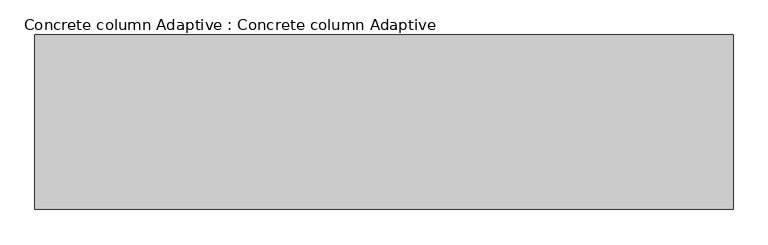
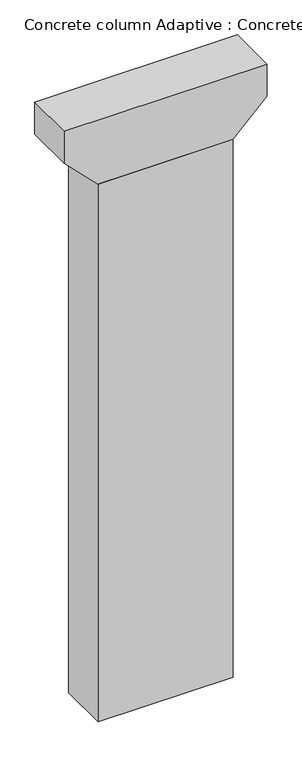
"""IFC4 building model written with IfcOpenShell, lengths in millimetres: proxy geometry, Concrete column Adaptive : Concrete column Adaptive."""

from ifc_helpers import new_model, si_unit, frame, origin, origin_with_axes, place, context, project, spatial, polyline, outline, extrude, source, transform, mapped, element, save


def concrete_column_adaptive_concrete_column_adaptive_f79cb2c7(model_context):
    return source(origin(), model_context, "Body", "SweptSolid", [
        extrude(outline(polyline([(37594.0, 6000.0), (37594.0, -6000.0), (35594.0, -6000.0), (33594.0, -4000.0), (33594.0, 4000.0), (35594.0, 6000.0), (37594.0, 6000.0)])), frame((0.0, -1500.0, 0.0), z_axis=(0.0, 1.0, 0.0), x_axis=(0.0, 0.0, 1.0)), (0.0, 0.0, 1.0), 3000.0),
        extrude(outline(polyline([(-4000.0, -1500.0), (-4000.0, 1500.0), (4000.0, 1500.0), (4000.0, -1500.0), (-4000.0, -1500.0)])), origin_with_axes(), (0.0, 0.0, 1.0), 33594.0),
    ])


if __name__ == "__main__":
    model = new_model("IFC4")
    model_context = context("Model", 3, world=origin())
    ifc_project = project(units=[si_unit("LENGTHUNIT", "METRE", prefix="MILLI")], contexts=[model_context])
    site = spatial("IfcSite", under=ifc_project)
    building = spatial("IfcBuilding", under=site)
    placement = place(None, origin())
    concrete_column_adaptive_concrete_column_adaptive_shape = concrete_column_adaptive_concrete_column_adaptive_f79cb2c7(model_context)
    element("IfcBuildingElementProxy", 1, Name="Concrete column Adaptive : Concrete column Adaptive", ObjectType="Concrete column Adaptive : Concrete column Adaptive", at=placement, inside=building, context=model_context, shape_type="MappedRepresentation", body=[
        mapped(concrete_column_adaptive_concrete_column_adaptive_shape, transform((0.0, 0.0, 0.0), x_axis=(1.0, 0.0, 0.0), y_axis=(0.0, 1.0, 0.0), z_axis=(0.0, 0.0, 1.0))),
    ])
    save(model, "model.ifc")

# Revit data of these elements
# Type "Concrete column Adaptive : Concrete column Adaptive"
#   Height [instance default] = 30000 mm
#   Default Elevation = 0
# Element 1 (IfcBuildingElementProxy, "Concrete column Adaptive : Concrete column Adaptive")
#   Height = 33594 mm
